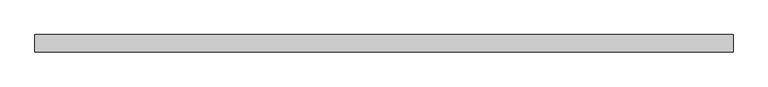
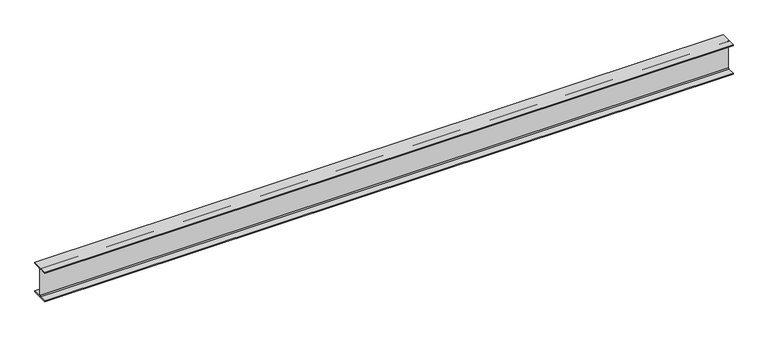
"""IFC4 building model written with IfcOpenShell, lengths in millimetres: beam geometry, Old_Steel Beam_H-KSD3502 : H_SB_ASB_H-340×250x9x14."""

from ifc_helpers import new_model, si_unit, point, frame, frame_2d, origin, place, context, project, spatial, polyline, circle_curve, trimmed, segment, composite_curve, outline, extrude, source, transform, mapped, element, save


def beam_59b3f42d(model_context):
    return source(origin(), model_context, "Body", "SweptSolid", [
        extrude(outline(composite_curve([segment(polyline([(82.5, -141.5), (82.5, -151.7), (-82.5, -151.7), (-82.5, -141.5), (-11.9, -141.5)]), True, "CONTINUOUS"), segment(trimmed(circle_curve(frame_2d((-11.9, -132.6)), 8.9), [point((-11.9, -141.5))], [point((-3.0, -132.6))], True, "CARTESIAN"), True, "CONTINUOUS"), segment(polyline([(-3.0, -132.6), (-3.0, 132.6)]), True, "CONTINUOUS"), segment(trimmed(circle_curve(frame_2d((-11.9, 132.6)), 8.9), [point((-3.0, 132.6))], [point((-11.9, 141.5))], True, "CARTESIAN"), True, "CONTINUOUS"), segment(polyline([(-11.9, 141.5), (-82.5, 141.5), (-82.5, 151.7), (82.5, 151.7), (82.5, 141.5), (11.9, 141.5)]), True, "CONTINUOUS"), segment(trimmed(circle_curve(frame_2d((11.9, 132.6)), 8.9), [point((11.9, 141.5))], [point((3.0, 132.6))], True, "CARTESIAN"), True, "CONTINUOUS"), segment(polyline([(3.0, 132.6), (3.0, -132.6)]), True, "CONTINUOUS"), segment(trimmed(circle_curve(frame_2d((11.9, -132.6)), 8.9), [point((3.0, -132.6))], [point((11.9, -141.5))], True, "CARTESIAN"), True, "CONTINUOUS"), segment(polyline([(11.9, -141.5), (82.5, -141.5)]), True, "CONTINUOUS")], self_intersect=False)), frame((-3337.3, 0.0, 0.0), z_axis=(1.0, 0.0, 0.0), x_axis=(0.0, 1.0, 0.0)), (0.0, 0.0, 1.0), 6674.6),
    ])


if __name__ == "__main__":
    model = new_model("IFC4")
    model_context = context("Model", 3, world=origin())
    ifc_project = project(units=[si_unit("LENGTHUNIT", "METRE", prefix="MILLI")], contexts=[model_context])
    site = spatial("IfcSite", under=ifc_project)
    building = spatial("IfcBuilding", under=site)
    placement = place(None, origin())
    beam_shape = beam_59b3f42d(model_context)
    element("IfcBeam", 1, ObjectType="Old_Steel Beam_H-KSD3502 : H_SB_ASB_H-340×250x9x14", at=placement, inside=building, context=model_context, shape_type="MappedRepresentation", body=[
        mapped(beam_shape, transform((0.0, 0.0, 0.0), x_axis=(1.0, 0.0, 0.0), y_axis=(0.0, 1.0, 0.0), z_axis=(0.0, 0.0, 1.0))),
    ])
    save(model, "model.ifc")

# Revit data of these elements
# Type "Old_Steel Beam_H-KSD3502 : H_SB_ASB_H-340×250x9x14"
#   Width = 25.0 cm
#   Web Thickness = 0.9 cm
#   Web Fillet = 2.0 cm
#   Warping Constant = 968661.0 cm⁶
#   Torsional Moment of Inertia = 53.6551 cm⁴
#   Torsional Modulus = 1.0 cm³
#   Section Area = 101.5 cm²
#   Plastic Modulus weak axis = 447.0 cm³
#   Plastic Modulus strong axis = 1410.0 cm³
#   Perimeter = 1.63 m²/m
#   Nominal Weight = 79.70 kgf/m
#   Moment of Inertia weak axis = 3650.00 cm⁴
#   Moment of Inertia strong axis = 21700.00 cm⁴
#   Height = 34.0 cm
#   Flange Thickness = 1.4 cm
#   Elastic Modulus weak axis = 292.0 cm³
#   Elastic Modulus strong axis = 1280.0 cm³
#   Centroid Vertical = 17.0 cm
#   Centroid Horizontal = 12.5 cm
#   Length [instance default] = 1.5240 m
#   Structural Material [instance default] = Steel, 45-345
#   Assembly Code = ""
# Element 1 (IfcBeam, "Old_Steel Beam_H-KSD3502 : H_SB_ASB_H-340×250x9x14")
#   Structural Material = none
# Materials
#   "Steel, 45-345": class "Metal", colour RGB 189 187 185, transparency 0, Description = "Steel 345 MPa", Cost = 0
